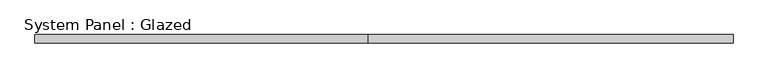
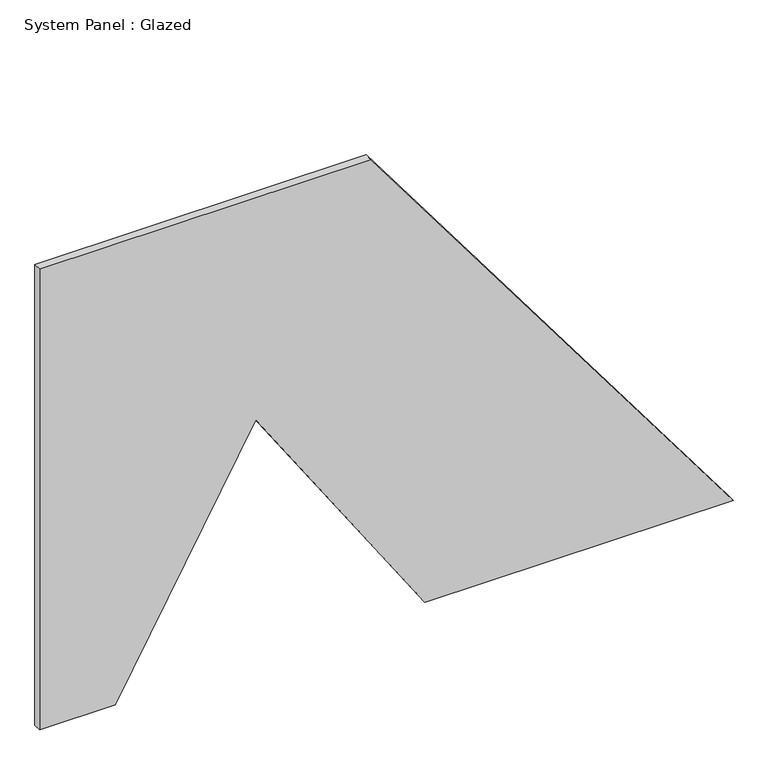
"""IFC4 building model written with IfcOpenShell, lengths in millimetres: plate geometry, System Panel : Glazed."""

import ifcopenshell
import ifcopenshell.guid

model = None  # the IFC model being written
_history = None  # IfcOwnerHistory: only IFC2X3 demands one
_inside = {}  # id of a spatial element -> (the spatial element, [elements in it])
_under = {}  # id of a project, library or spatial element -> (it, [spatial elements below it])
_declared = {}  # id of a project -> (the project, [libraries it declares])
_typed = {}  # id of a type object -> (the type object, [elements of that type])
_made_of = {}  # id of a material, layer set ... -> (it, [elements and type objects made of it])


def new_model(schema):
    """Start an empty IFC model of exactly this schema.

    Asked for "IFC4X3", IfcOpenShell would pick the latest addendum, in which some entities
    have other attributes; the version numbers below select the first issue.
    IFC2X3 requires an IfcOwnerHistory on every rooted entity: one is made here for all.
    """
    global model, _history
    if schema == "IFC4X3":
        model = ifcopenshell.file(schema_version=(4, 3, 0, 0))
    else:
        model = ifcopenshell.file(schema=schema)
    _inside.clear()
    _under.clear()
    _declared.clear()
    _typed.clear()
    _made_of.clear()
    _history = None
    if model.schema == "IFC2X3":
        org = make("IfcOrganization", Name="unknown")
        user = make(
            "IfcPersonAndOrganization",
            ThePerson=make("IfcPerson", FamilyName="unknown"),
            TheOrganization=org,
        )
        app = make(
            "IfcApplication",
            ApplicationDeveloper=org,
            Version="unknown",
            ApplicationFullName="unknown",
            ApplicationIdentifier="unknown",
        )
        _history = make(
            "IfcOwnerHistory",
            OwningUser=user,
            OwningApplication=app,
            ChangeAction="ADDED",
            CreationDate=0,
        )
    return model


def make(cls, **values):
    """One entity of the class cls with the attributes given. An attribute that is None is left unset."""
    return model.create_entity(
        cls, **{name: value for name, value in values.items() if value is not None}
    )


def rooted(cls, **values):
    """An entity with a GlobalId (a new one), such as an element, a storey or a relation."""
    return make(cls, GlobalId=ifcopenshell.guid.new(), OwnerHistory=_history, **values)


def si_unit(unit_type, name, prefix=None):
    """IfcSIUnit, for example si_unit("LENGTHUNIT", "METRE", prefix="MILLI")."""
    return make("IfcSIUnit", UnitType=unit_type, Prefix=prefix, Name=name)


def assignment(units):
    """IfcUnitAssignment: the units of a project."""
    return None if units is None else make("IfcUnitAssignment", Units=units)


def point(xyz):
    """IfcCartesianPoint."""
    return None if xyz is None else make("IfcCartesianPoint", Coordinates=xyz)


def direction(xyz):
    """IfcDirection."""
    return None if xyz is None else make("IfcDirection", DirectionRatios=xyz)


def frame(location, z_axis=None, x_axis=None):
    """IfcAxis2Placement3D, a coordinate frame: its origin and axes. An axis left out is left unset."""
    return make(
        "IfcAxis2Placement3D",
        Location=point(location),
        Axis=direction(z_axis),
        RefDirection=direction(x_axis),
    )


def origin():
    """The frame at (0, 0, 0) with its axes left unset."""
    return frame((0.0, 0.0, 0.0))


def place(relative_to, where):
    """IfcLocalPlacement: puts the frame where relative to a parent placement (None: the world)."""
    return make(
        "IfcLocalPlacement", PlacementRelTo=relative_to, RelativePlacement=where
    )


def context(
    kind, dimensions, precision=None, world=None, true_north=None, identifier=None
):
    """IfcGeometricRepresentationContext, for example the 3D "Model" context."""
    return make(
        "IfcGeometricRepresentationContext",
        ContextIdentifier=identifier,
        ContextType=kind,
        CoordinateSpaceDimension=dimensions,
        Precision=precision,
        WorldCoordinateSystem=world,
        TrueNorth=true_north,
    )


def project(units=None, contexts=None):
    """IfcProject with its units and contexts."""
    return rooted(
        "IfcProject",
        Name="project",
        RepresentationContexts=contexts,
        UnitsInContext=assignment(units),
    )


def spatial(cls, under=None, at=None, **own):
    """A site, building, storey or space (cls), placed at a placement, below another one or the project."""
    s = rooted(cls, ObjectPlacement=at, **own)
    if under is not None:
        _under.setdefault(under.id(), (under, []))[1].append(s)
    return s


def polyline(points):
    """IfcPolyline through the points."""
    return make("IfcPolyline", Points=[point(p) for p in points])


def outline(outer, holes=None, kind="AREA"):
    """IfcArbitraryClosedProfileDef: a profile drawn as a closed curve; with holes, ...WithVoids."""
    if holes is None:
        return make("IfcArbitraryClosedProfileDef", ProfileType=kind, OuterCurve=outer)
    return make(
        "IfcArbitraryProfileDefWithVoids",
        ProfileType=kind,
        OuterCurve=outer,
        InnerCurves=holes,
    )


def extrude(swept, where, along, depth):
    """IfcExtrudedAreaSolid: the profile swept, set in the frame where, extruded along a direction by depth."""
    return make(
        "IfcExtrudedAreaSolid",
        SweptArea=swept,
        Position=where,
        ExtrudedDirection=direction(along),
        Depth=depth,
    )


def shape(context_of_items, identifier, shape_type, items):
    """IfcShapeRepresentation: the items that make up one representation, for example the "Body"."""
    return make(
        "IfcShapeRepresentation",
        ContextOfItems=context_of_items,
        RepresentationIdentifier=identifier,
        RepresentationType=shape_type,
        Items=items,
    )


def source(mapping_origin, context_of_items, identifier, shape_type, items):
    """IfcRepresentationMap: a shape defined once, which mapped items show again and again."""
    return make(
        "IfcRepresentationMap",
        MappingOrigin=mapping_origin,
        MappedRepresentation=shape(context_of_items, identifier, shape_type, items),
    )


def transform(
    local_origin,
    x_axis=None,
    y_axis=None,
    z_axis=None,
    scale=None,
    scale2=None,
    scale3=None,
    uniform=True,
):
    """IfcCartesianTransformationOperator3D, or its non-uniform kind. x_axis, y_axis, z_axis: its Axis1, 2, 3."""
    if uniform:
        return make(
            "IfcCartesianTransformationOperator3D",
            Axis1=direction(x_axis),
            Axis2=direction(y_axis),
            LocalOrigin=point(local_origin),
            Scale=scale,
            Axis3=direction(z_axis),
        )
    return make(
        "IfcCartesianTransformationOperator3DnonUniform",
        Axis1=direction(x_axis),
        Axis2=direction(y_axis),
        LocalOrigin=point(local_origin),
        Scale=scale,
        Axis3=direction(z_axis),
        Scale2=scale2,
        Scale3=scale3,
    )


def mapped(mapping_source, mapping_target):
    """IfcMappedItem: shows the shape of a source again, moved by a transform."""
    return make(
        "IfcMappedItem", MappingSource=mapping_source, MappingTarget=mapping_target
    )


def made_of(thing, what):
    """Note that an element or type object is made of a material, layer set ...; save() writes the relation."""
    if what is not None:
        _made_of.setdefault(what.id(), (what, []))[1].append(thing)
    return thing


def element(
    cls,
    number,
    at=None,
    inside=None,
    cuts=None,
    type_object=None,
    material=None,
    context=None,
    identifier="Body",
    shape_type=None,
    held_by="IfcProductDefinitionShape",
    body=None,
    shapes=None,
    **own,
):
    """One element of the class cls, such as IfcWall. Its Tag is "e" and its number.

    at: its placement. inside: the storey or other place that contains it. cuts: it is an
    opening in that element (IfcRelVoidsElement). A single representation is given by context,
    identifier, shape_type and body (its items); several are given by shapes. held_by: the class
    of the entity that holds the representations. save() writes the other relations.
    """
    e = rooted(cls, Tag="e%d" % number, ObjectPlacement=at, **own)
    if body is not None:
        shapes = [shape(context, identifier, shape_type, body)]
    if shapes is not None:
        e.Representation = make(held_by, Representations=shapes)
    if inside is not None:
        _inside.setdefault(inside.id(), (inside, []))[1].append(e)
    if cuts is not None:
        rooted(
            "IfcRelVoidsElement", RelatingBuildingElement=cuts, RelatedOpeningElement=e
        )
    if type_object is not None:
        _typed.setdefault(type_object.id(), (type_object, []))[1].append(e)
    return made_of(e, material)


def aggregate(whole, parts):
    """IfcRelAggregates: a whole, such as a stair, and the parts it consists of."""
    return rooted("IfcRelAggregates", RelatingObject=whole, RelatedObjects=parts)


def save(model, path):
    """Write the relations noted so far, then the file.

    IfcRelAggregates (storeys below a building ...), IfcRelContainedInSpatialStructure (elements
    in a storey), IfcRelDefinesByType, IfcRelAssociatesMaterial and IfcRelDeclares: one each for
    every whole, place, type object, material and project.
    """
    for whole, parts in _under.values():
        aggregate(whole, parts)
    for where, things in _inside.values():
        rooted(
            "IfcRelContainedInSpatialStructure",
            RelatedElements=things,
            RelatingStructure=where,
        )
    for kind, things in _typed.values():
        rooted("IfcRelDefinesByType", RelatedObjects=things, RelatingType=kind)
    for what, things in _made_of.values():
        rooted("IfcRelAssociatesMaterial", RelatedObjects=things, RelatingMaterial=what)
    for by, libraries in _declared.values():
        rooted("IfcRelDeclares", RelatingContext=by, RelatedDefinitions=libraries)
    model.write(path)


def system_panel_glazed_62d74c5f(model_context):
    return source(origin(), model_context, "Body", "SweptSolid", [
        extrude(outline(polyline([(0.0, -1067.2452277), (0.0, -834.2633716), (775.7163604, -401.9930078), (0.0, 118.6994992), (0.0, 1067.2452277), (1500.0, -47.6081203), (1500.0, -1067.2452277), (0.0, -1067.2452277)])), frame((0.0, 24.5, 0.0), z_axis=(0.0, 1.0, 0.0), x_axis=(0.0, 0.0, 1.0)), (0.0, 0.0, 1.0), 25.0),
    ])


if __name__ == "__main__":
    model = new_model("IFC4")
    model_context = context("Model", 3, world=origin())
    ifc_project = project(units=[si_unit("LENGTHUNIT", "METRE", prefix="MILLI")], contexts=[model_context])
    site = spatial("IfcSite", under=ifc_project)
    building = spatial("IfcBuilding", under=site)
    placement = place(None, origin())
    system_panel_glazed_shape = system_panel_glazed_62d74c5f(model_context)
    element("IfcPlate", 1, ObjectType="System Panel : Glazed", at=placement, inside=building, context=model_context, shape_type="MappedRepresentation", body=[
        mapped(system_panel_glazed_shape, transform((0.0, 0.0, 0.0), x_axis=(1.0, 0.0, 0.0), y_axis=(0.0, 1.0, 0.0), z_axis=(0.0, 0.0, 1.0))),
    ])
    save(model, "model.ifc")

# Revit data of these elements
# Type "System Panel : Glazed"
#   Construction Type Id = "GSP4R"
#   Analytic Construction = "1/8 in Pilkington single glazing"
#   Visual Light Transmittance = 0.9
#   Solar Heat Gain Coefficient = 0.86
#   Heat Transfer Coefficient (U) = 6.7069 W/(m²·K)
#   Define Thermal Properties by = 1
# Element 1 (IfcPlate, "System Panel : Glazed")
#   Materials on its faces: "Glass"
# Materials
#   "Glass": class "Glass", colour RGB 0 128 192, transparency 0.9, Description = "Soda Lime Glass", Cost = 0
